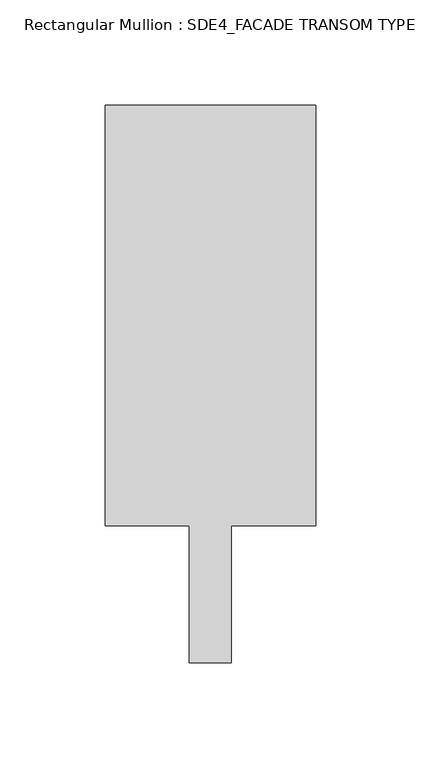
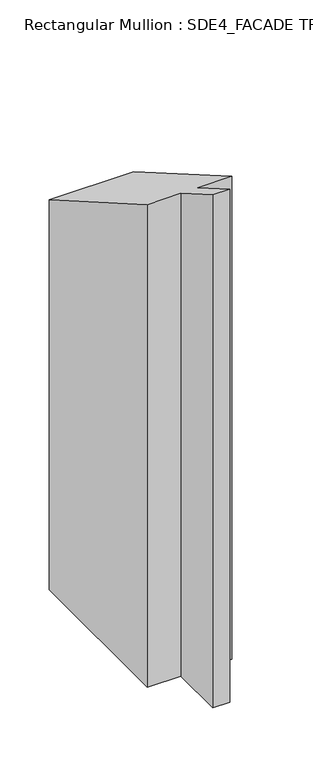
"""IFC4 building model written with IfcOpenShell, lengths in millimetres: member geometry, Rectangular Mullion : SDE4_FACADE TRANSOM TYPE 2."""

from ifc_helpers import new_model, si_unit, origin, place, context, project, spatial, faceted_brep, source, transform, mapped, element, save


def rectangular_mullion_sde4_facade_transom_type_2_f7e526c2(model_context):
    return source(origin(), model_context, "Body", "Brep", [
        faceted_brep([(50.0, 132.5, -562.3560667), (50.0, -67.5, -562.3560667), (10.0, -67.5, -562.3560667), (10.0, -132.5, -562.3560667), (-10.0, -132.5, -562.3560667), (-10.0, -67.5, -562.3560667), (-50.0, -67.5, -562.3560667), (-50.0, 132.5, -562.3560667), (-50.0, 132.5, -76.4361394), (50.0, 132.5, -76.4361394), (-50.0, -67.5, 38.9391654), (-10.0, -67.5, 38.9391654), (-10.0, -132.5, 76.4361394), (10.0, -132.5, 76.4361394), (10.0, -67.5, 38.9391654), (50.0, -67.5, 38.9391654)], [[[0, 1, 2, 3, 4, 5, 6, 7]], [[8, 9, 0, 7]], [[10, 8, 7, 6]], [[11, 10, 6, 5]], [[12, 11, 5, 4]], [[13, 12, 4, 3]], [[14, 13, 3, 2]], [[15, 14, 2, 1]], [[9, 15, 1, 0]], [[9, 8, 10, 11, 12, 13, 14, 15]]]),
    ])


if __name__ == "__main__":
    model = new_model("IFC4")
    model_context = context("Model", 3, world=origin())
    ifc_project = project(units=[si_unit("LENGTHUNIT", "METRE", prefix="MILLI")], contexts=[model_context])
    site = spatial("IfcSite", under=ifc_project)
    building = spatial("IfcBuilding", under=site)
    placement = place(None, origin())
    rectangular_mullion_sde4_facade_transom_type_2_shape = rectangular_mullion_sde4_facade_transom_type_2_f7e526c2(model_context)
    element("IfcMember", 1, ObjectType="Rectangular Mullion : SDE4_FACADE TRANSOM TYPE 2", at=placement, inside=building, context=model_context, shape_type="MappedRepresentation", body=[
        mapped(rectangular_mullion_sde4_facade_transom_type_2_shape, transform((0.0, 0.0, 0.0), x_axis=(1.0, 0.0, 0.0), y_axis=(0.0, 1.0, 0.0), z_axis=(0.0, 0.0, 1.0))),
    ])
    save(model, "model.ifc")

# Revit data of these elements
# Type "Rectangular Mullion : SDE4_FACADE TRANSOM TYPE 2"
#   built-in parameter 1007322 = 0.869423 (stored number, unit not read)
#   built-in parameter 1007321 = 0.164042 (stored number, unit not read)
#   built-in parameter 1007320 = 0.164042 (stored number, unit not read)
